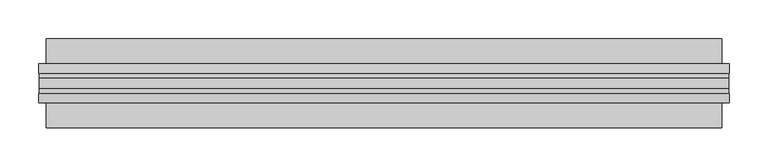
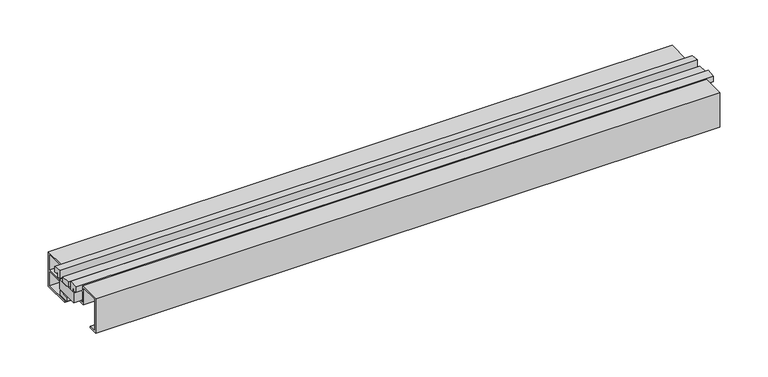
"""IFC4 building model written with IfcOpenShell, lengths in millimetres: proxy geometry, Generic Models 3:Generic Models 1:2:Generic Models 1:2 : Generic Models 3:Generic Models 1:300625:328150:Generic Models 1:2:Generic Models 1:2 : Generic Models 3:Generic Models 1:300625:328150 : Generic Models 3:Generic Models 1:2:Generic Models 1:2 : Generic Models 3:Generic Models 1:300625:328150:6 : Generic Models 3:Generic Models 1:2:Generic Models 1:2 : Generic Models 3:Generic Models 1:300625:328150:Generic Models 1:2:Generic Models 1:2 : Generic Models 3:Generic Models 1:300625:328150 : Generic Models 3:Generic Models 1:2:Generic Models 1:2 : Generic Models 3:Generic Models 1:300625:328150:300962."""

from ifc_helpers import new_model, si_unit, frame, origin, place, context, project, spatial, polyline, outline, extrude, source, transform, mapped, element, save


def generic_models_393137f4(model_context):
    return source(origin(), model_context, "Body", "SweptSolid", [
        extrude(outline(polyline([(593690.1661787, -579047.2017564), (593690.1661787, -579080.4885915), (592803.3447692, -579080.4885915), (592803.3447692, -579047.2017564), (593690.1661787, -579047.2017564)])), frame((0.0, 0.0, 56.1634725), z_axis=(0.0, 0.0, 1.0), x_axis=(1.0, 0.0, 0.0)), (0.0, 0.0, 1.0), 14.2115027),
        extrude(outline(polyline([(593690.1661787, -579047.8857325), (593690.1661787, -579063.9971687), (592803.3447692, -579063.9971687), (592803.3447692, -579047.8857325), (593690.1661787, -579047.8857325)])), frame((0.0, 0.0, 48.1837518), z_axis=(0.0, 0.0, 1.0), x_axis=(1.0, 0.0, 0.0)), (0.0, 0.0, 1.0), 6.0797872),
        extrude(outline(polyline([(593690.1661787, -579054.6663841), (593690.1661787, -579067.3832724), (592803.3447692, -579067.3832724), (592803.3447692, -579054.6663841), (593690.1661787, -579054.6663841)])), frame((0.0, 0.0, 70.3749752), z_axis=(0.0, 0.0, 1.0), x_axis=(1.0, 0.0, 0.0)), (0.0, 0.0, 1.0), 8.3194793),
        extrude(outline(polyline([(-579078.8757591, 77.6675716), (-579081.7214373, 77.6675716), (-579081.7214373, 74.7237119), (-579086.0195091, 74.7237119), (-579086.0195091, 82.5634213), (-579074.1217032, 84.0242882), (-579074.1217032, 71.954031), (-579078.8757591, 71.954031), (-579078.8757591, 77.6675716)])), frame((592802.9478941, 0.0, 0.0), z_axis=(1.0, 0.0, 0.0), x_axis=(0.0, 1.0, 0.0)), (0.0, 0.0, 1.0), 887.6151596),
        extrude(outline(polyline([(-579036.0470357, 82.5634213), (-579036.0470357, 74.7237119), (-579040.3451075, 74.7237119), (-579040.3451075, 77.6675716), (-579043.1907857, 77.6675716), (-579043.1907857, 71.954031), (-579047.9448415, 71.954031), (-579047.9448415, 84.0242882), (-579036.0470357, 82.5634213)])), frame((592802.9478941, 0.0, 0.0), z_axis=(1.0, 0.0, 0.0), x_axis=(0.0, 1.0, 0.0)), (0.0, 0.0, 1.0), 887.6151596),
        extrude(outline(polyline([(-579118.1663841, 30.7803608), (-579118.1663841, 81.5465842), (-579086.4163841, 81.5465842), (-579086.4163841, 74.3268369), (-579081.3245623, 74.3268369), (-579081.3245623, 77.2706967), (-579079.2726341, 77.2706967), (-579079.2726341, 72.350906), (-579086.4163841, 72.350906), (-579086.4163841, 56.1634725), (-579059.1333389, 56.1634725), (-579059.1333389, 54.263539), (-579063.9971687, 54.263539), (-579063.9971687, 48.1837518), (-579059.1333389, 48.1837518), (-579059.1333389, 46.891797), (-579065.8971022, 46.891797), (-579065.8971022, 54.263539), (-579088.3163176, 54.263539), (-579088.3163176, 79.6466507), (-579115.6584719, 79.6466507), (-579115.6584719, 32.6802943), (-579105.079253, 32.6802943), (-579105.079253, 30.7803608), (-579118.1663841, 30.7803608)])), frame((592812.5404473, 0.0, 0.0), z_axis=(1.0, 0.0, 0.0), x_axis=(0.0, 1.0, 0.0)), (0.0, 0.0, 1.0), 868.4300532),
        extrude(outline(polyline([(-579040.7419825, 77.2706967), (-579040.7419825, 74.3268369), (-579035.6501607, 74.3268369), (-579035.6501607, 81.5465842), (-579003.8663841, 81.5465842), (-579003.8663841, 30.7803608), (-579042.7939107, 30.7803608), (-579042.7939107, 32.7025734), (-579005.8423149, 32.7025734), (-579005.8423149, 54.263539), (-579045.985799, 54.263539), (-579045.985799, 46.891797), (-579052.7495623, 46.891797), (-579052.7495623, 48.1837518), (-579047.8857325, 48.1837518), (-579047.8857325, 54.263539), (-579052.7495623, 54.263539), (-579052.7495623, 56.1634725), (-579005.8423149, 56.1634725), (-579005.8423149, 79.6367852), (-579033.7502272, 79.6367852), (-579033.7502272, 72.350906), (-579042.7939107, 72.350906), (-579042.7939107, 77.2706967), (-579040.7419825, 77.2706967)])), frame((592812.5404473, 0.0, 0.0), z_axis=(1.0, 0.0, 0.0), x_axis=(0.0, 1.0, 0.0)), (0.0, 0.0, 1.0), 868.4300532),
    ])


if __name__ == "__main__":
    model = new_model("IFC4")
    model_context = context("Model", 3, world=origin())
    ifc_project = project(units=[si_unit("LENGTHUNIT", "METRE", prefix="MILLI")], contexts=[model_context])
    site = spatial("IfcSite", under=ifc_project)
    building = spatial("IfcBuilding", under=site)
    placement = place(None, origin())
    generic_models_shape = generic_models_393137f4(model_context)
    element("IfcBuildingElementProxy", 1, Name="Generic Models 3:Generic Models 1:2:Generic Models 1:2 : Generic Models 3:Generic Models 1:300625:328150:Generic Models 1:2:Generic Models 1:2 : Generic Models 3:Generic Models 1:300625:328150 : Generic Models 3:Generic Models 1:2:Generic Models 1:2 : Generic Models 3:Generic Models 1:300625:328150:6 : Generic Models 3:Generic Models 1:2:Generic Models 1:2 : Generic Models 3:Generic Models 1:300625:328150:Generic Models 1:2:Generic Models 1:2 : Generic Models 3:Generic Models 1:300625:328150 : Generic Models 3:Generic Models 1:2:Generic Models 1:2 : Generic Models 3:Generic Models 1:300625:328150:300962", ObjectType="Generic Models 3:Generic Models 1:2:Generic Models 1:2 : Generic Models 3:Generic Models 1:300625:328150:Generic Models 1:2:Generic Models 1:2 : Generic Models 3:Generic Models 1:300625:328150 : Generic Models 3:Generic Models 1:2:Generic Models 1:2 : Generic Models 3:Generic Models 1:300625:328150:6 : Generic Models 3:Generic Models 1:2:Generic Models 1:2 : Generic Models 3:Generic Models 1:300625:328150:Generic Models 1:2:Generic Models 1:2 : Generic Models 3:Generic Models 1:300625:328150 : Generic Models 3:Generic Models 1:2:Generic Models 1:2 : Generic Models 3:Generic Models 1:300625:328150:300962", at=placement, inside=building, context=model_context, shape_type="MappedRepresentation", body=[
        mapped(generic_models_shape, transform((0.0, 0.0, 0.0), x_axis=(1.0, 0.0, 0.0), y_axis=(0.0, 1.0, 0.0), z_axis=(0.0, 0.0, 1.0))),
    ])
    save(model, "model.ifc")

# Revit data of these elements
# Type "Generic Models 3:Generic Models 1:2:Generic Models 1:2 : Generic Models 3:Generic Models 1:300625:328150:Generic Models 1:2:Generic Models 1:2 : Generic Models 3:Generic Models 1:300625:328150 : Generic Models 3:Generic Models 1:2:Generic Models 1:2 : Generic Models 3:Generic Models 1:300625:328150:6 : Generic Models 3:Generic Models 1:2:Generic Models 1:2 : Generic Models 3:Generic Models 1:300625:328150:Generic Models 1:2:Generic Models 1:2 : Generic Models 3:Generic Models 1:300625:328150 : Generic Models 3:Generic Models 1:2:Generic Models 1:2 : Generic Models 3:Generic Models 1:300625:328150:300962"
#   NameOverride = "Generic Models 3:Generic Models 1:2:Generic Models 1:2 : Generic Models 3:Generic Models 1:300625:328150:Generic Models 1:2:Generic Models 1:2 : Generic Models 3:Generic Models 1:300625:328150 : Generic Models 3:Generic Models 1:2:Generic Models 1:2 : Generic Models 3:Generic Models 1:300625:328150:300962"
#   ObjectTypeOverride = "Generic Models 1:2:Generic Models 1:2 : Generic Models 3:Generic Models 1:300625:328150 : Generic Models 3:Generic Models 1:2:Generic Models 1:2 : Generic Models 3:Generic Models 1:300625:328150"
#   Reference = "Generic Models 1"
#   Tag = "300962"
# Element 1 (IfcBuildingElementProxy, "Generic Models 3:Generic Models 1:2:Generic Models 1:2 : Generic Models 3:Generic Models 1:300625:328150:Generic Models 1:2:Generic Models 1:2 : Generic Models 3:Generic Models 1:300625:328150 : Generic Models 3:Generic Models 1:2:Generic Models 1:2 : Generic Models 3:Generic Models 1:300625:328150:6 : Generic Models 3:Generic Models 1:2:Generic Models 1:2 : Generic Models 3:Generic Models 1:300625:328150:Generic Models 1:2:Generic Models 1:2 : Generic Models 3:Generic Models 1:300625:328150 : Generic Models 3:Generic Models 1:2:Generic Models 1:2 : Generic Models 3:Generic Models 1:300625:328150:300962")
#   Materials on its faces: "THERMAL BROKEN ALUMINUM STOREFRONT"
# Materials
#   "THERMAL BROKEN ALUMINUM STOREFRONT": class "Unassigned", colour RGB 244 244 244, transparency 0, Cost = 0
